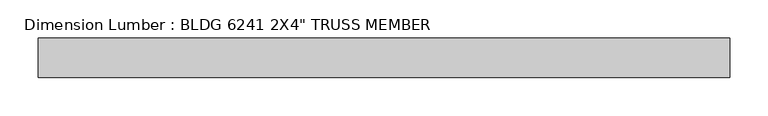
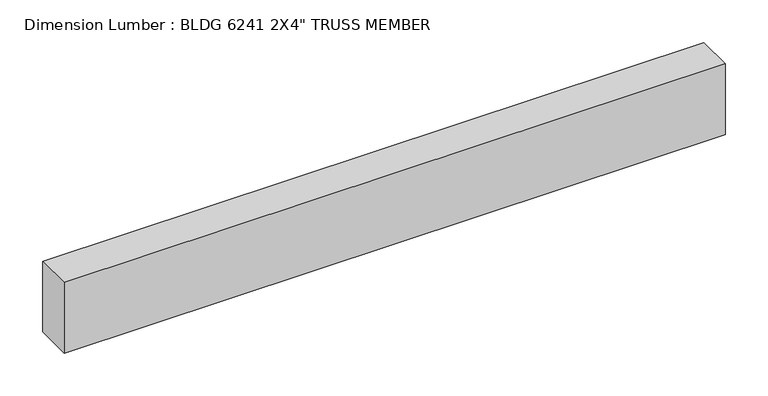
"""IFC4 building model written with IfcOpenShell, lengths in millimetres: beam geometry."""

from ifc_helpers import new_model, si_unit, frame, origin, place, context, project, spatial, polyline, outline, extrude, source, transform, mapped, element, save


def beam_4e9e3d70(model_context):
    return source(origin(), model_context, "Body", "SweptSolid", [
        extrude(outline(polyline([(492.3733183, 25.4), (492.3733183, -25.4), (-405.6522938, -25.4), (-405.6522938, 25.4), (492.3733183, 25.4)])), frame((0.0, 0.0, -50.8), z_axis=(0.0, 0.0, 1.0), x_axis=(1.0, 0.0, 0.0)), (0.0, 0.0, 1.0), 101.6),
    ])


if __name__ == "__main__":
    model = new_model("IFC4")
    model_context = context("Model", 3, world=origin())
    ifc_project = project(units=[si_unit("LENGTHUNIT", "METRE", prefix="MILLI")], contexts=[model_context])
    site = spatial("IfcSite", under=ifc_project)
    building = spatial("IfcBuilding", under=site)
    placement = place(None, origin())
    beam_shape = beam_4e9e3d70(model_context)
    element("IfcBeam", 1, ObjectType="Dimension Lumber : BLDG 6241 2X4\" TRUSS MEMBER", at=placement, inside=building, context=model_context, shape_type="MappedRepresentation", body=[
        mapped(beam_shape, transform((0.0, 0.0, 0.0), x_axis=(1.0, 0.0, 0.0), y_axis=(0.0, 1.0, 0.0), z_axis=(0.0, 0.0, 1.0))),
    ])
    save(model, "model.ifc")

# Revit data of these elements
# Type "Dimension Lumber : BLDG 6241 2X4\" TRUSS MEMBER"
#   Assembly Code = "B10"
#   A = 0.273472 SF
#   Length [instance default] = 5' - 0"
#   b = 0' - 2"
#   d = 0' - 4"
#   Structural Material [instance default] = Softwood, Lumber
# Element 1 (IfcBeam, "Dimension Lumber : BLDG 6241 2X4\" TRUSS MEMBER")
#   Materials on its faces: "Softwood, Lumber"
# Materials
#   "Softwood, Lumber": class "Wood", colour RGB 223 192 134, transparency 0, Description = "Pinus Echinata", Cost = 0
